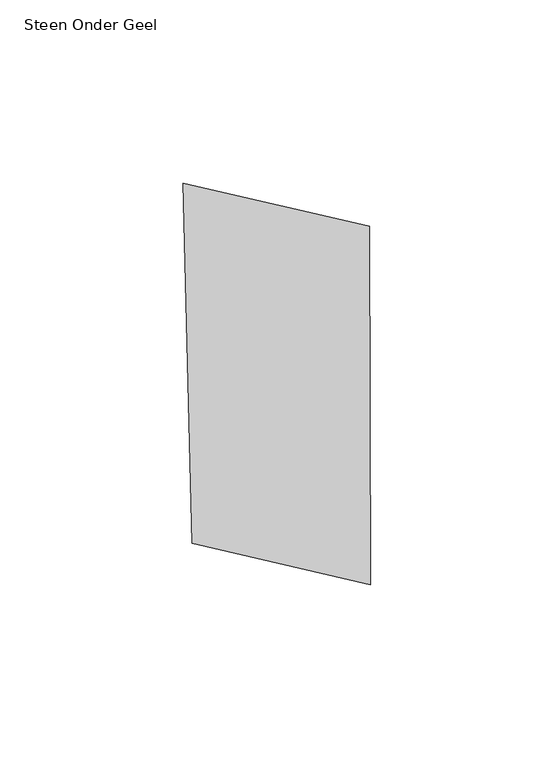
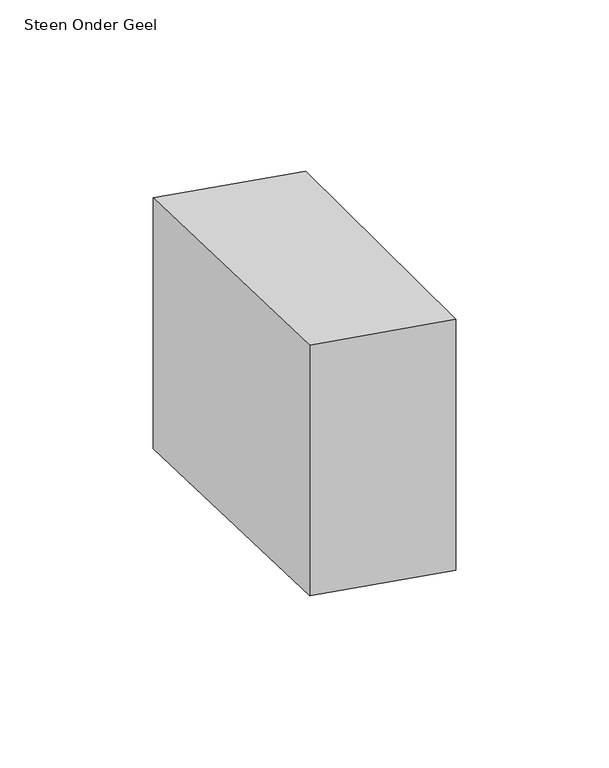
"""IFC4 building model written with IfcOpenShell, lengths in millimetres: proxy geometry, 00_GMA_steen_versie_4 : Steen Onder Geel."""

from ifc_helpers import new_model, si_unit, origin, origin_with_axes, place, context, project, spatial, polyline, outline, extrude, source, transform, mapped, element, save


def steen_onder_geel_e16bfb8f(model_context):
    return source(origin(), model_context, "Body", "SweptSolid", [
        extrude(outline(polyline([(100.5337327, 116.0617811), (100.8432702, 18.3741751), (52.1154016, 29.5810844), (49.7441134, 127.7643021), (100.5337327, 116.0617811)])), origin_with_axes(), (0.0, 0.0, 1.0), 100.0),
    ])


if __name__ == "__main__":
    model = new_model("IFC4")
    model_context = context("Model", 3, world=origin())
    ifc_project = project(units=[si_unit("LENGTHUNIT", "METRE", prefix="MILLI")], contexts=[model_context])
    site = spatial("IfcSite", under=ifc_project)
    building = spatial("IfcBuilding", under=site)
    placement = place(None, origin())
    steen_onder_geel_shape = steen_onder_geel_e16bfb8f(model_context)
    element("IfcBuildingElementProxy", 1, Name="00_GMA_steen_versie_4 : Steen Onder Geel", ObjectType="00_GMA_steen_versie_4 : Steen Onder Geel", at=placement, inside=building, context=model_context, shape_type="MappedRepresentation", body=[
        mapped(steen_onder_geel_shape, transform((0.0, 0.0, 0.0), x_axis=(1.0, 0.0, 0.0), y_axis=(0.0, 1.0, 0.0), z_axis=(0.0, 0.0, 1.0))),
    ])
    save(model, "model.ifc")

# Revit data of these elements
# Type "00_GMA_steen_versie_4 : Steen Onder Geel"
#   StootVoegHalfBoven [instance default] = 5 mm
#   StootVoegHalf [instance default] = 5 mm
#   StootVoegBreedteOnder = 10 mm
#   StootVoegBreedteBoven = 10 mm
#   Steendikte = 100 mm
#   LintVoegOnderHalf = 0 mm
#   LintVoegOnder = 0 mm
#   LintVoegBovenHalf = 5 mm
#   LintVoegBoven = 10 mm
#   materiaal = 21_steen_geel
#   MateriaalVoeg = none
#   Default Elevation = 0
# Element 1 (IfcBuildingElementProxy, "00_GMA_steen_versie_4 : Steen Onder Geel")
#   Materials on its faces: "21_steen_geel"
# Materials
#   "21_steen_geel": class "Unassigned", colour RGB 202 202 0, transparency 0, Cost = 0
